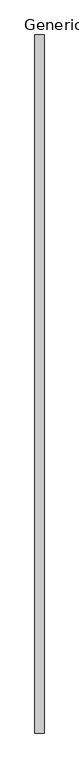
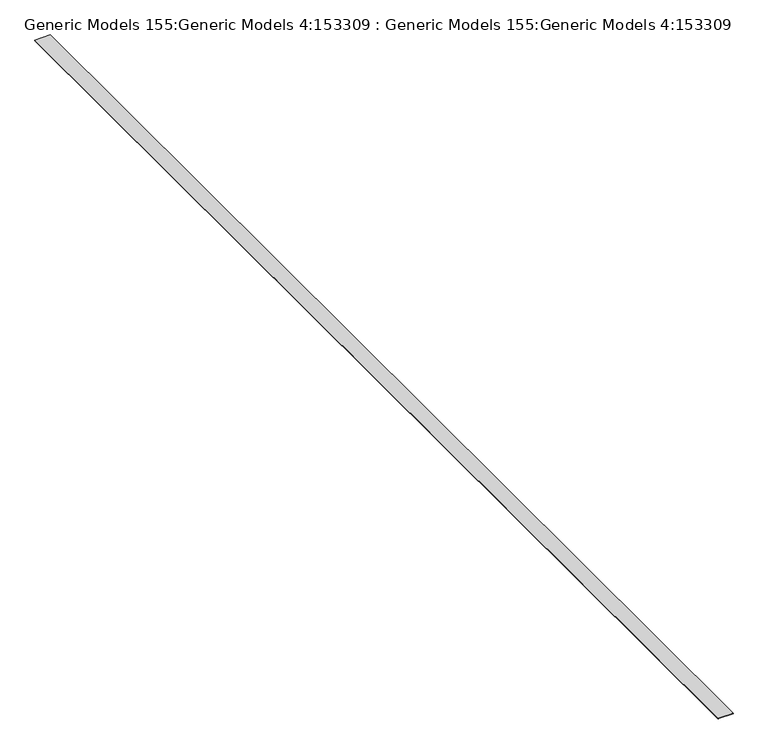
"""IFC4 building model written with IfcOpenShell, lengths in millimetres: proxy geometry, Generic Models 155:Generic Models 4:153309 : Generic Models 155:Generic Models 4:153309."""

from ifc_helpers import new_model, si_unit, frame, origin, place, context, project, spatial, polyline, outline, extrude, source, transform, mapped, element, save


def generic_models_155_generic_models_4_153309_generic_models_c4e23679(model_context):
    return source(origin(), model_context, "Body", "SweptSolid", [
        extrude(outline(polyline([(-6544.9716051, 2583.5025207), (-6544.9716051, -5303.1974793), (-6648.131089, -5303.1974793), (-6648.131089, 2583.5025207), (-6544.9716051, 2583.5025207)])), frame((0.0, 0.0, -33.7996684), z_axis=(0.0, 0.0, 1.0), x_axis=(1.0, 0.0, 0.0)), (0.0, 0.0, 1.0), 1.3753749),
        extrude(outline(polyline([(-6544.9716051, 2583.5025207), (-6544.9716051, -5303.1974793), (-6648.131089, -5303.1974793), (-6648.131089, 2583.5025207), (-6544.9716051, 2583.5025207)])), frame((0.0, 0.0, -37.1933267), z_axis=(0.0, 0.0, 1.0), x_axis=(1.0, 0.0, 0.0)), (0.0, 0.0, 1.0), 1.3753749),
    ])


if __name__ == "__main__":
    model = new_model("IFC4")
    model_context = context("Model", 3, world=origin())
    ifc_project = project(units=[si_unit("LENGTHUNIT", "METRE", prefix="MILLI")], contexts=[model_context])
    site = spatial("IfcSite", under=ifc_project)
    building = spatial("IfcBuilding", under=site)
    placement = place(None, origin())
    generic_models_155_generic_models_4_153309_generic_models_shape = generic_models_155_generic_models_4_153309_generic_models_c4e23679(model_context)
    element("IfcBuildingElementProxy", 1, Name="Generic Models 155:Generic Models 4:153309 : Generic Models 155:Generic Models 4:153309", ObjectType="Generic Models 155:Generic Models 4:153309 : Generic Models 155:Generic Models 4:153309", at=placement, inside=building, context=model_context, shape_type="MappedRepresentation", body=[
        mapped(generic_models_155_generic_models_4_153309_generic_models_shape, transform((0.0, 0.0, 0.0), x_axis=(1.0, 0.0, 0.0), y_axis=(0.0, 1.0, 0.0), z_axis=(0.0, 0.0, 1.0))),
    ])
    save(model, "model.ifc")

# Revit data of these elements
# Type "Generic Models 155:Generic Models 4:153309 : Generic Models 155:Generic Models 4:153309"
#   NameOverride = "Generic Models 155:Generic Models 4:153309"
#   ObjectTypeOverride = "Generic Models 155:Generic Models 4"
#   Reference = "Generic Models 4"
#   Category = "Generic Models"
#   Tag = "153309"
# Element 1 (IfcBuildingElementProxy, "Generic Models 155:Generic Models 4:153309 : Generic Models 155:Generic Models 4:153309")
#   Materials on its faces: "_BED OF SEALANT (ABOVE/BELOW FLASHING) 12592"
# Materials
#   "_BED OF SEALANT (ABOVE/BELOW FLASHING) 12592": class "Unassigned", colour RGB 253 192 103, transparency 0
